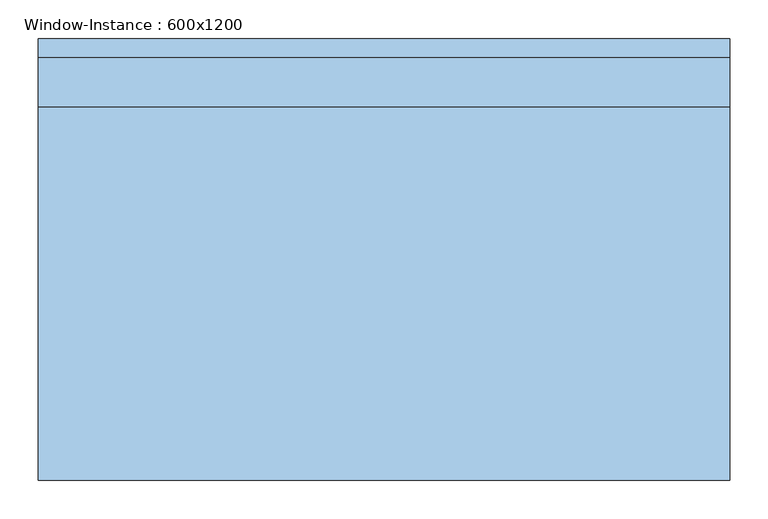
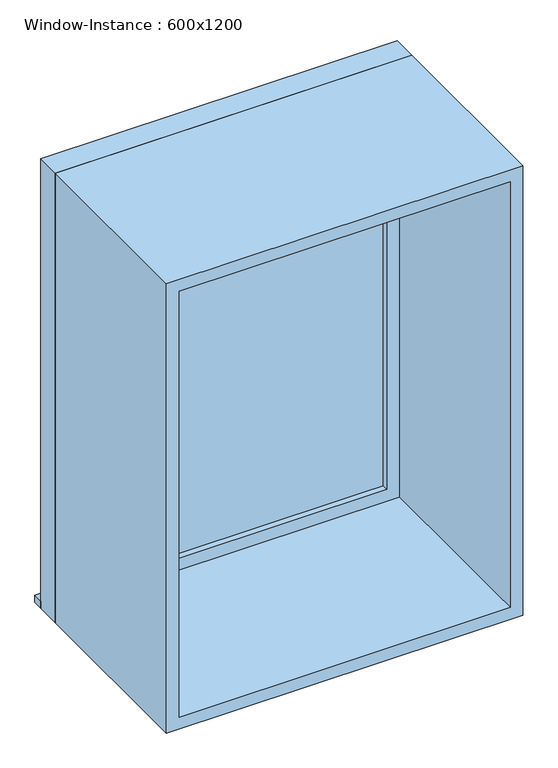
"""IFC4 building model written with IfcOpenShell, lengths in millimetres: window geometry, Window-Instance : 600x1200."""

import ifcopenshell
import ifcopenshell.guid

model = None  # the IFC model being written
_history = None  # IfcOwnerHistory: only IFC2X3 demands one
_inside = {}  # id of a spatial element -> (the spatial element, [elements in it])
_under = {}  # id of a project, library or spatial element -> (it, [spatial elements below it])
_declared = {}  # id of a project -> (the project, [libraries it declares])
_typed = {}  # id of a type object -> (the type object, [elements of that type])
_made_of = {}  # id of a material, layer set ... -> (it, [elements and type objects made of it])


def new_model(schema):
    """Start an empty IFC model of exactly this schema.

    Asked for "IFC4X3", IfcOpenShell would pick the latest addendum, in which some entities
    have other attributes; the version numbers below select the first issue.
    IFC2X3 requires an IfcOwnerHistory on every rooted entity: one is made here for all.
    """
    global model, _history
    if schema == "IFC4X3":
        model = ifcopenshell.file(schema_version=(4, 3, 0, 0))
    else:
        model = ifcopenshell.file(schema=schema)
    _inside.clear()
    _under.clear()
    _declared.clear()
    _typed.clear()
    _made_of.clear()
    _history = None
    if model.schema == "IFC2X3":
        org = make("IfcOrganization", Name="unknown")
        user = make(
            "IfcPersonAndOrganization",
            ThePerson=make("IfcPerson", FamilyName="unknown"),
            TheOrganization=org,
        )
        app = make(
            "IfcApplication",
            ApplicationDeveloper=org,
            Version="unknown",
            ApplicationFullName="unknown",
            ApplicationIdentifier="unknown",
        )
        _history = make(
            "IfcOwnerHistory",
            OwningUser=user,
            OwningApplication=app,
            ChangeAction="ADDED",
            CreationDate=0,
        )
    return model


def make(cls, **values):
    """One entity of the class cls with the attributes given. An attribute that is None is left unset."""
    return model.create_entity(
        cls, **{name: value for name, value in values.items() if value is not None}
    )


def rooted(cls, **values):
    """An entity with a GlobalId (a new one), such as an element, a storey or a relation."""
    return make(cls, GlobalId=ifcopenshell.guid.new(), OwnerHistory=_history, **values)


def si_unit(unit_type, name, prefix=None):
    """IfcSIUnit, for example si_unit("LENGTHUNIT", "METRE", prefix="MILLI")."""
    return make("IfcSIUnit", UnitType=unit_type, Prefix=prefix, Name=name)


def assignment(units):
    """IfcUnitAssignment: the units of a project."""
    return None if units is None else make("IfcUnitAssignment", Units=units)


def point(xyz):
    """IfcCartesianPoint."""
    return None if xyz is None else make("IfcCartesianPoint", Coordinates=xyz)


def direction(xyz):
    """IfcDirection."""
    return None if xyz is None else make("IfcDirection", DirectionRatios=xyz)


def frame(location, z_axis=None, x_axis=None):
    """IfcAxis2Placement3D, a coordinate frame: its origin and axes. An axis left out is left unset."""
    return make(
        "IfcAxis2Placement3D",
        Location=point(location),
        Axis=direction(z_axis),
        RefDirection=direction(x_axis),
    )


def origin():
    """The frame at (0, 0, 0) with its axes left unset."""
    return frame((0.0, 0.0, 0.0))


def place(relative_to, where):
    """IfcLocalPlacement: puts the frame where relative to a parent placement (None: the world)."""
    return make(
        "IfcLocalPlacement", PlacementRelTo=relative_to, RelativePlacement=where
    )


def context(
    kind, dimensions, precision=None, world=None, true_north=None, identifier=None
):
    """IfcGeometricRepresentationContext, for example the 3D "Model" context."""
    return make(
        "IfcGeometricRepresentationContext",
        ContextIdentifier=identifier,
        ContextType=kind,
        CoordinateSpaceDimension=dimensions,
        Precision=precision,
        WorldCoordinateSystem=world,
        TrueNorth=true_north,
    )


def project(units=None, contexts=None):
    """IfcProject with its units and contexts."""
    return rooted(
        "IfcProject",
        Name="project",
        RepresentationContexts=contexts,
        UnitsInContext=assignment(units),
    )


def spatial(cls, under=None, at=None, **own):
    """A site, building, storey or space (cls), placed at a placement, below another one or the project."""
    s = rooted(cls, ObjectPlacement=at, **own)
    if under is not None:
        _under.setdefault(under.id(), (under, []))[1].append(s)
    return s


def polyline(points):
    """IfcPolyline through the points."""
    return make("IfcPolyline", Points=[point(p) for p in points])


def outline(outer, holes=None, kind="AREA"):
    """IfcArbitraryClosedProfileDef: a profile drawn as a closed curve; with holes, ...WithVoids."""
    if holes is None:
        return make("IfcArbitraryClosedProfileDef", ProfileType=kind, OuterCurve=outer)
    return make(
        "IfcArbitraryProfileDefWithVoids",
        ProfileType=kind,
        OuterCurve=outer,
        InnerCurves=holes,
    )


def extrude(swept, where, along, depth):
    """IfcExtrudedAreaSolid: the profile swept, set in the frame where, extruded along a direction by depth."""
    return make(
        "IfcExtrudedAreaSolid",
        SweptArea=swept,
        Position=where,
        ExtrudedDirection=direction(along),
        Depth=depth,
    )


def shape(context_of_items, identifier, shape_type, items):
    """IfcShapeRepresentation: the items that make up one representation, for example the "Body"."""
    return make(
        "IfcShapeRepresentation",
        ContextOfItems=context_of_items,
        RepresentationIdentifier=identifier,
        RepresentationType=shape_type,
        Items=items,
    )


def source(mapping_origin, context_of_items, identifier, shape_type, items):
    """IfcRepresentationMap: a shape defined once, which mapped items show again and again."""
    return make(
        "IfcRepresentationMap",
        MappingOrigin=mapping_origin,
        MappedRepresentation=shape(context_of_items, identifier, shape_type, items),
    )


def transform(
    local_origin,
    x_axis=None,
    y_axis=None,
    z_axis=None,
    scale=None,
    scale2=None,
    scale3=None,
    uniform=True,
):
    """IfcCartesianTransformationOperator3D, or its non-uniform kind. x_axis, y_axis, z_axis: its Axis1, 2, 3."""
    if uniform:
        return make(
            "IfcCartesianTransformationOperator3D",
            Axis1=direction(x_axis),
            Axis2=direction(y_axis),
            LocalOrigin=point(local_origin),
            Scale=scale,
            Axis3=direction(z_axis),
        )
    return make(
        "IfcCartesianTransformationOperator3DnonUniform",
        Axis1=direction(x_axis),
        Axis2=direction(y_axis),
        LocalOrigin=point(local_origin),
        Scale=scale,
        Axis3=direction(z_axis),
        Scale2=scale2,
        Scale3=scale3,
    )


def mapped(mapping_source, mapping_target):
    """IfcMappedItem: shows the shape of a source again, moved by a transform."""
    return make(
        "IfcMappedItem", MappingSource=mapping_source, MappingTarget=mapping_target
    )


def made_of(thing, what):
    """Note that an element or type object is made of a material, layer set ...; save() writes the relation."""
    if what is not None:
        _made_of.setdefault(what.id(), (what, []))[1].append(thing)
    return thing


def element(
    cls,
    number,
    at=None,
    inside=None,
    cuts=None,
    type_object=None,
    material=None,
    context=None,
    identifier="Body",
    shape_type=None,
    held_by="IfcProductDefinitionShape",
    body=None,
    shapes=None,
    **own,
):
    """One element of the class cls, such as IfcWall. Its Tag is "e" and its number.

    at: its placement. inside: the storey or other place that contains it. cuts: it is an
    opening in that element (IfcRelVoidsElement). A single representation is given by context,
    identifier, shape_type and body (its items); several are given by shapes. held_by: the class
    of the entity that holds the representations. save() writes the other relations.
    """
    e = rooted(cls, Tag="e%d" % number, ObjectPlacement=at, **own)
    if body is not None:
        shapes = [shape(context, identifier, shape_type, body)]
    if shapes is not None:
        e.Representation = make(held_by, Representations=shapes)
    if inside is not None:
        _inside.setdefault(inside.id(), (inside, []))[1].append(e)
    if cuts is not None:
        rooted(
            "IfcRelVoidsElement", RelatingBuildingElement=cuts, RelatedOpeningElement=e
        )
    if type_object is not None:
        _typed.setdefault(type_object.id(), (type_object, []))[1].append(e)
    return made_of(e, material)


def aggregate(whole, parts):
    """IfcRelAggregates: a whole, such as a stair, and the parts it consists of."""
    return rooted("IfcRelAggregates", RelatingObject=whole, RelatedObjects=parts)


def save(model, path):
    """Write the relations noted so far, then the file.

    IfcRelAggregates (storeys below a building ...), IfcRelContainedInSpatialStructure (elements
    in a storey), IfcRelDefinesByType, IfcRelAssociatesMaterial and IfcRelDeclares: one each for
    every whole, place, type object, material and project.
    """
    for whole, parts in _under.values():
        aggregate(whole, parts)
    for where, things in _inside.values():
        rooted(
            "IfcRelContainedInSpatialStructure",
            RelatedElements=things,
            RelatingStructure=where,
        )
    for kind, things in _typed.values():
        rooted("IfcRelDefinesByType", RelatedObjects=things, RelatingType=kind)
    for what, things in _made_of.values():
        rooted("IfcRelAssociatesMaterial", RelatedObjects=things, RelatingMaterial=what)
    for by, libraries in _declared.values():
        rooted("IfcRelDeclares", RelatingContext=by, RelatedDefinitions=libraries)
    model.write(path)


def window_instance_600x1200_0f68ffda(model_context):
    return source(origin(), model_context, "Body", "SweptSolid", [
        extrude(outline(polyline([(-488.1, 300.4), (411.9, 300.4), (411.9, 275.0), (-488.1, 275.0), (-488.1, 300.4)])), frame((0.0, 0.0, 900.0), z_axis=(0.0, 0.0, 1.0), x_axis=(1.0, 0.0, 0.0)), (0.0, 0.0, 1.0), 19.05),
        extrude(outline(polyline([(348.4, 226.425), (-424.6, 226.425), (-424.6, 239.125), (348.4, 239.125), (348.4, 226.425)])), frame((0.0, 0.0, 963.5), z_axis=(0.0, 0.0, 1.0), x_axis=(1.0, 0.0, 0.0)), (0.0, 0.0, 1.0), 1073.0),
        extrude(outline(polyline([(2080.95, -469.05), (919.05, -469.05), (919.05, 392.85), (2080.95, 392.85), (2080.95, -469.05)]), holes=[polyline([(2036.5, -424.6), (2036.5, 348.4), (963.5, 348.4), (963.5, -424.6), (2036.5, -424.6)])]), frame((0.0, 210.55, 0.0), z_axis=(0.0, 1.0, 0.0), x_axis=(0.0, 0.0, 1.0)), (0.0, 0.0, 1.0), 44.45),
        extrude(outline(polyline([(2100.0, -488.1), (900.0, -488.1), (900.0, 411.9), (2100.0, 411.9), (2100.0, -488.1)]), holes=[polyline([(2068.25, -456.35), (2068.25, 380.15), (931.75, 380.15), (931.75, -456.35), (2068.25, -456.35)])]), frame((0.0, -275.0, 0.0), z_axis=(0.0, 1.0, 0.0), x_axis=(0.0, 0.0, 1.0)), (0.0, 0.0, 1.0), 485.55),
        extrude(outline(polyline([(2100.0, 411.9), (2100.0, -488.1), (900.0, -488.1), (900.0, 411.9), (2100.0, 411.9)]), holes=[polyline([(2080.95, 392.85), (919.05, 392.85), (919.05, -469.05), (2080.95, -469.05), (2080.95, 392.85)])]), frame((0.0, 210.55, 0.0), z_axis=(0.0, 1.0, 0.0), x_axis=(0.0, 0.0, 1.0)), (0.0, 0.0, 1.0), 64.45),
    ])


if __name__ == "__main__":
    model = new_model("IFC4")
    model_context = context("Model", 3, world=origin())
    ifc_project = project(units=[si_unit("LENGTHUNIT", "METRE", prefix="MILLI")], contexts=[model_context])
    site = spatial("IfcSite", under=ifc_project)
    building = spatial("IfcBuilding", under=site)
    placement = place(None, origin())
    window_instance_600x1200_shape = window_instance_600x1200_0f68ffda(model_context)
    element("IfcWindow", 1, ObjectType="Window-Instance : 600x1200", at=placement, inside=building, context=model_context, shape_type="MappedRepresentation", body=[
        mapped(window_instance_600x1200_shape, transform((0.0, 0.0, 0.0), x_axis=(1.0, 0.0, 0.0), y_axis=(0.0, 1.0, 0.0), z_axis=(0.0, 0.0, 1.0))),
    ])
    save(model, "model.ifc")

# Revit data of these elements
# Type "Window-Instance : 600x1200"
#   Type Mark = "7"
#   Construction Type Id = "GSP4R"
#   Assembly Code = "B2020100"
#   Analytic Construction = "1/8 in Pilkington single glazing"
#   Visual Light Transmittance = 0.9
#   Thermal Resistance (R) = 0.149095 (m²·K)/W
#   Solar Heat Gain Coefficient = 0.86
#   Heat Transfer Coefficient (U) = 6.70716 W/(m²·K)
#   Height [instance default] = 1200 mm
#   Default Sill Height = 900 mm
#   Width [instance default] = 600 mm
#   Window Inset = 20 mm
#   Glass Pane Material = WW-EC-GL-Storefront
#   Sash Material = WW-EC-RGB-White
#   Wall Closure = (empty or 0)
# Element 1 (IfcWindow, "Window-Instance : 600x1200")
#   Width = 900 mm
#   Materials on its faces: "WW-EC-RGB-White", "WW-EC-GL-Storefront"
# Materials
#   "WW-EC-GL-Storefront": class "Glass", colour RGB 236 240 239, transparency 0.85, Description = "Storefront Glass", Cost = 0
#   "WW-EC-RGB-White": class "Generic", colour RGB 255 255 255, transparency 0, Comments = "If region requests off-white, swith asset color to RGB 231-228-220", Description = "Generic Color", Cost = 0
